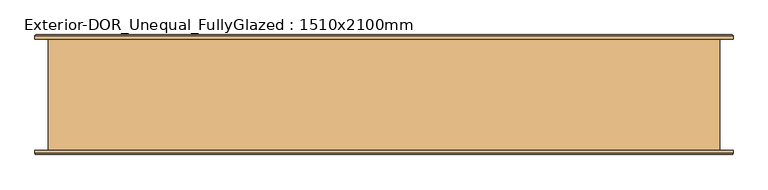
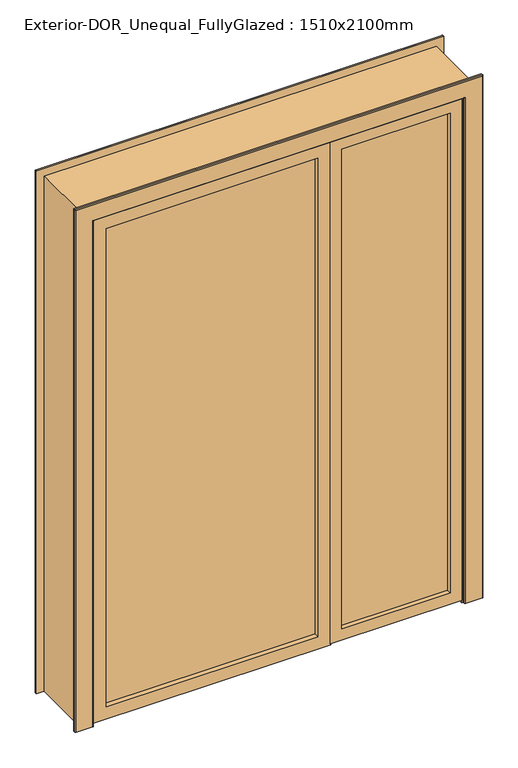
"""IFC4 building model written with IfcOpenShell, lengths in millimetres: door geometry, Exterior-DOR_Unequal_FullyGlazed : 1510x2100mm."""

from ifc_helpers import new_model, si_unit, frame, origin, place, context, project, spatial, polyline, circle_curve, ellipse_curve, outline, extrude, faceted_brep, source, transform, mapped, element, save
from ifc_brep_helpers import plane_surface, cylinder_surface, advanced_brep


def exterior_dor_unequal_fullyglazed_1510x2100mm_99816280(model_context):
    return source(origin(), model_context, "Body", "SolidModel", [
        extrude(outline(polyline([(247.5, -106.0), (247.5, -99.0), (665.0, -99.0), (665.0, -106.0), (247.5, -106.0)])), frame((0.0, 0.0, 55.0), z_axis=(0.0, 0.0, 1.0), x_axis=(1.0, 0.0, 0.0)), (0.0, 0.0, 1.0), 1955.0),
        extrude(outline(polyline([(10.0, 710.0), (2055.0, 710.0), (2055.0, 202.5), (10.0, 202.5), (10.0, 710.0)]), holes=[polyline([(2010.0, 247.5), (2010.0, 665.0), (55.0, 665.0), (55.0, 247.5), (2010.0, 247.5)])]), frame((0.0, -125.0, 0.0), z_axis=(0.0, 1.0, 0.0), x_axis=(0.0, 0.0, 1.0)), (0.0, 0.0, 1.0), 45.0),
        extrude(outline(polyline([(155.0, -106.0), (-660.0, -106.0), (-660.0, -99.0), (155.0, -99.0), (155.0, -106.0)])), frame((0.0, 0.0, 56.0), z_axis=(0.0, 0.0, 1.0), x_axis=(1.0, 0.0, 0.0)), (0.0, 0.0, 1.0), 1949.0),
        extrude(outline(polyline([(6.0, -710.0), (6.0, 205.0), (2055.0, 205.0), (2055.0, -710.0), (6.0, -710.0)]), holes=[polyline([(2005.0, 155.0), (56.0, 155.0), (56.0, -660.0), (2005.0, -660.0), (2005.0, 155.0)])]), frame((0.0, -125.0, 0.0), z_axis=(0.0, 1.0, 0.0), x_axis=(0.0, 0.0, 1.0)), (0.0, 0.0, 1.0), 45.0),
        advanced_brep(
        [(-715.0, -125.0, 0.0), (-715.0, -132.0, 0.0), (-718.0, -135.0, 0.0), (-782.0, -135.0, 0.0), (-785.0, -132.0, 0.0), (-785.0, -125.0, 0.0), (-715.0, -125.0, 2060.0), (-715.0, -132.0, 2060.0), (-718.0, -135.0, 2063.0), (718.0, -135.0, 2063.0), (718.0, -135.0, 0.0), (782.0, -135.0, 0.0), (782.0, -135.0, 2127.0), (-782.0, -135.0, 2127.0), (-785.0, -132.0, 2130.0), (-785.0, -125.0, 2130.0), (785.0, -125.0, 2130.0), (785.0, -125.0, 0.0), (715.0, -125.0, 0.0), (715.0, -125.0, 2060.0), (715.0, -132.0, 2060.0), (715.0, -132.0, 0.0), (785.0, -132.0, 0.0), (785.0, -132.0, 2130.0)],
        [
            (0, 1),
            (1, 2, circle_curve(frame((-718.0, -132.0, 0.0), z_axis=(0.0, 0.0, -1.0), x_axis=(-1.0, 0.0, 0.0)), 3.0)),
            (2, 3),
            (3, 4, circle_curve(frame((-782.0, -132.0, 0.0), z_axis=(0.0, 0.0, -1.0), x_axis=(-1.0, 0.0, 0.0)), 3.0)),
            (4, 5),
            (5, 0),
            (0, 6),
            (6, 7),
            (7, 1),
            (7, 8, ellipse_curve(frame((-718.0, -132.0, 2063.0), z_axis=(-0.7071067811865475, 0.0, -0.7071067811865475), x_axis=(0.7071067811865474, 0.0, -0.7071067811865476)), 4.2426407, 3.0)),
            (8, 2),
            (8, 9),
            (9, 10),
            (10, 11),
            (11, 12),
            (12, 13),
            (13, 3),
            (13, 14, ellipse_curve(frame((-782.0, -132.0, 2127.0), z_axis=(-0.7071067811865475, 0.0, -0.7071067811865475), x_axis=(0.7071067811865474, 0.0, -0.7071067811865476)), 4.2426407, 3.0)),
            (14, 4),
            (14, 15),
            (15, 5),
            (15, 16),
            (16, 17),
            (17, 18),
            (18, 19),
            (19, 6),
            (9, 20, ellipse_curve(frame((718.0, -132.0, 2063.0), z_axis=(0.7071067811865475, 0.0, -0.7071067811865475), x_axis=(0.7071067811865474, 0.0, 0.7071067811865476)), 4.2426407, 3.0)),
            (20, 21),
            (21, 10, circle_curve(frame((718.0, -132.0, 0.0), z_axis=(0.0, 0.0, 1.0), x_axis=(1.0, 0.0, 0.0)), 3.0)),
            (17, 22),
            (22, 11, circle_curve(frame((782.0, -132.0, 0.0), z_axis=(0.0, 0.0, -1.0), x_axis=(1.0, 0.0, 0.0)), 3.0)),
            (21, 18),
            (23, 12, ellipse_curve(frame((782.0, -132.0, 2127.0), z_axis=(0.7071067811865475, 0.0, -0.7071067811865475), x_axis=(0.7071067811865474, 0.0, 0.7071067811865476)), 4.2426407, 3.0)),
            (22, 23),
            (16, 23),
            (20, 19),
            (20, 7),
            (23, 14),
        ],
        [
            plane_surface(frame((-755.0, 125.0, 0.0), z_axis=(0.0, 0.0, -1.0), x_axis=(0.0, -1.0, 0.0))),
            plane_surface(frame((-715.0, -125.0, 0.0), z_axis=(1.0, 0.0, 0.0), x_axis=(0.0, 0.0, 1.0))),
            cylinder_surface(frame((-718.0, -132.0, 0.0), z_axis=(0.0, 0.0, -1.0), x_axis=(-1.0, 0.0, 0.0)), 3.0),
            plane_surface(frame((-718.0, -135.0, 0.0), z_axis=(0.0, -1.0, 0.0), x_axis=(0.0, 0.0, 1.0))),
            cylinder_surface(frame((-782.0, -132.0, 0.0), z_axis=(0.0, 0.0, -1.0), x_axis=(-1.0, 0.0, 0.0)), 3.0),
            plane_surface(frame((-785.0, -132.0, 0.0), z_axis=(-1.0, 0.0, 0.0), x_axis=(0.0, 0.0, 1.0))),
            plane_surface(frame((-785.0, -125.0, 0.0), z_axis=(0.0, 1.0, 0.0), x_axis=(0.0, 0.0, 1.0))),
            cylinder_surface(frame((718.0, -132.0, 2100.0), z_axis=(0.0, 0.0, 1.0), x_axis=(1.0, 0.0, 0.0)), 3.0),
            plane_surface(frame((755.0, 125.0, 0.0), z_axis=(0.0, 0.0, -1.0), x_axis=(0.0, -1.0, 0.0))),
            cylinder_surface(frame((782.0, -132.0, 2100.0), z_axis=(0.0, 0.0, 1.0), x_axis=(1.0, 0.0, 0.0)), 3.0),
            plane_surface(frame((785.0, -132.0, 2130.0), z_axis=(1.0, 0.0, 0.0), x_axis=(0.0, 0.0, -1.0))),
            plane_surface(frame((715.0, -125.0, 2060.0), z_axis=(-1.0, 0.0, 0.0), x_axis=(0.0, 0.0, -1.0))),
            plane_surface(frame((-715.0, -125.0, 2060.0), z_axis=(0.0, 0.0, -1.0), x_axis=(1.0, 0.0, 0.0))),
            cylinder_surface(frame((-755.0, -132.0, 2063.0), z_axis=(-1.0, 0.0, 0.0), x_axis=(0.0, 0.0, 1.0)), 3.0),
            cylinder_surface(frame((-755.0, -132.0, 2127.0), z_axis=(-1.0, 0.0, 0.0), x_axis=(0.0, 0.0, 1.0)), 3.0),
            plane_surface(frame((-785.0, -132.0, 2130.0), z_axis=(0.0, 0.0, 1.0), x_axis=(1.0, 0.0, 0.0))),
        ],
        [
            (0, [[1, 2, 3, 4, 5, 6]]),
            (1, [[-1, 7, 8, 9]]),
            (2, [[-2, -9, 10, 11]]),
            (3, [[-3, -11, 12, 13, 14, 15, 16, 17]]),
            (4, [[-4, -17, 18, 19]]),
            (5, [[-5, -19, 20, 21]]),
            (6, [[-6, -21, 22, 23, 24, 25, 26, -7]]),
            (7, [[27, 28, 29, -13]]),
            (8, [[-24, 30, 31, -14, -29, 32]]),
            (9, [[33, -15, -31, 34]]),
            (10, [[35, -34, -30, -23]]),
            (11, [[36, -25, -32, -28]]),
            (12, [[-8, -26, -36, 37]]),
            (13, [[-10, -37, -27, -12]]),
            (14, [[-18, -16, -33, 38]]),
            (15, [[-20, -38, -35, -22]]),
        ],
    ),
        advanced_brep(
        [(-785.0, 125.0, 0.0), (-785.0, 132.0, 0.0), (-782.0, 135.0, 0.0), (-718.0, 135.0, 0.0), (-715.0, 132.0, 0.0), (-715.0, 125.0, 0.0), (-785.0, 125.0, 2130.0), (-785.0, 132.0, 2130.0), (-782.0, 135.0, 2127.0), (782.0, 135.0, 2127.0), (782.0, 135.0, 0.0), (718.0, 135.0, 0.0), (718.0, 135.0, 2063.0), (-718.0, 135.0, 2063.0), (-715.0, 132.0, 2060.0), (-715.0, 125.0, 2060.0), (715.0, 125.0, 2060.0), (715.0, 125.0, 0.0), (785.0, 125.0, 0.0), (785.0, 125.0, 2130.0), (785.0, 132.0, 2130.0), (785.0, 132.0, 0.0), (715.0, 132.0, 0.0), (715.0, 132.0, 2060.0)],
        [
            (0, 1),
            (1, 2, circle_curve(frame((-782.0, 132.0, 0.0), z_axis=(0.0, 0.0, -1.0), x_axis=(-1.0, 0.0, 0.0)), 3.0)),
            (2, 3),
            (3, 4, circle_curve(frame((-718.0, 132.0, 0.0), z_axis=(0.0, 0.0, -1.0), x_axis=(-1.0, 0.0, 0.0)), 3.0)),
            (4, 5),
            (5, 0),
            (0, 6),
            (6, 7),
            (7, 1),
            (7, 8, ellipse_curve(frame((-782.0, 132.0, 2127.0), z_axis=(-0.7071067811865475, 0.0, -0.7071067811865475), x_axis=(0.7071067811865474, 0.0, -0.7071067811865476)), 4.2426407, 3.0)),
            (8, 2),
            (8, 9),
            (9, 10),
            (10, 11),
            (11, 12),
            (12, 13),
            (13, 3),
            (13, 14, ellipse_curve(frame((-718.0, 132.0, 2063.0), z_axis=(-0.7071067811865475, 0.0, -0.7071067811865475), x_axis=(0.7071067811865474, 0.0, -0.7071067811865476)), 4.2426407, 3.0)),
            (14, 4),
            (14, 15),
            (15, 5),
            (15, 16),
            (16, 17),
            (17, 18),
            (18, 19),
            (19, 6),
            (9, 20, ellipse_curve(frame((782.0, 132.0, 2127.0), z_axis=(0.7071067811865475, 0.0, -0.7071067811865475), x_axis=(0.7071067811865474, 0.0, 0.7071067811865476)), 4.2426407, 3.0)),
            (20, 21),
            (21, 10, circle_curve(frame((782.0, 132.0, 0.0), z_axis=(0.0, 0.0, 1.0), x_axis=(1.0, 0.0, 0.0)), 3.0)),
            (17, 22),
            (22, 11, circle_curve(frame((718.0, 132.0, 0.0), z_axis=(0.0, 0.0, -1.0), x_axis=(1.0, 0.0, 0.0)), 3.0)),
            (21, 18),
            (23, 12, ellipse_curve(frame((718.0, 132.0, 2063.0), z_axis=(0.7071067811865475, 0.0, -0.7071067811865475), x_axis=(0.7071067811865474, 0.0, 0.7071067811865476)), 4.2426407, 3.0)),
            (22, 23),
            (16, 23),
            (20, 19),
            (20, 7),
            (23, 14),
        ],
        [
            plane_surface(frame((-755.0, 125.0, 0.0), z_axis=(0.0, 0.0, -1.0), x_axis=(0.0, -1.0, 0.0))),
            plane_surface(frame((-785.0, 125.0, 0.0), z_axis=(-1.0, 0.0, 0.0), x_axis=(0.0, 0.0, 1.0))),
            cylinder_surface(frame((-782.0, 132.0, 0.0), z_axis=(0.0, 0.0, -1.0), x_axis=(-1.0, 0.0, 0.0)), 3.0),
            plane_surface(frame((-782.0, 135.0, 0.0), z_axis=(0.0, 1.0, 0.0), x_axis=(0.0, 0.0, 1.0))),
            cylinder_surface(frame((-718.0, 132.0, 0.0), z_axis=(0.0, 0.0, -1.0), x_axis=(-1.0, 0.0, 0.0)), 3.0),
            plane_surface(frame((-715.0, 132.0, 0.0), z_axis=(1.0, 0.0, 0.0), x_axis=(0.0, 0.0, 1.0))),
            plane_surface(frame((-715.0, 125.0, 0.0), z_axis=(0.0, -1.0, 0.0), x_axis=(0.0, 0.0, 1.0))),
            cylinder_surface(frame((782.0, 132.0, 2100.0), z_axis=(0.0, 0.0, 1.0), x_axis=(1.0, 0.0, 0.0)), 3.0),
            plane_surface(frame((755.0, 125.0, 0.0), z_axis=(0.0, 0.0, -1.0), x_axis=(0.0, -1.0, 0.0))),
            cylinder_surface(frame((718.0, 132.0, 2100.0), z_axis=(0.0, 0.0, 1.0), x_axis=(1.0, 0.0, 0.0)), 3.0),
            plane_surface(frame((715.0, 132.0, 2060.0), z_axis=(-1.0, 0.0, 0.0), x_axis=(0.0, 0.0, -1.0))),
            plane_surface(frame((785.0, 125.0, 2130.0), z_axis=(1.0, 0.0, 0.0), x_axis=(0.0, 0.0, -1.0))),
            plane_surface(frame((-785.0, 125.0, 2130.0), z_axis=(0.0, 0.0, 1.0), x_axis=(1.0, 0.0, 0.0))),
            cylinder_surface(frame((-755.0, 132.0, 2127.0), z_axis=(-1.0, 0.0, 0.0), x_axis=(0.0, 0.0, 1.0)), 3.0),
            cylinder_surface(frame((-755.0, 132.0, 2063.0), z_axis=(-1.0, 0.0, 0.0), x_axis=(0.0, 0.0, 1.0)), 3.0),
            plane_surface(frame((-715.0, 132.0, 2060.0), z_axis=(0.0, 0.0, -1.0), x_axis=(1.0, 0.0, 0.0))),
        ],
        [
            (0, [[1, 2, 3, 4, 5, 6]]),
            (1, [[-1, 7, 8, 9]]),
            (2, [[-2, -9, 10, 11]]),
            (3, [[-3, -11, 12, 13, 14, 15, 16, 17]]),
            (4, [[-4, -17, 18, 19]]),
            (5, [[-5, -19, 20, 21]]),
            (6, [[-6, -21, 22, 23, 24, 25, 26, -7]]),
            (7, [[27, 28, 29, -13]]),
            (8, [[-24, 30, 31, -14, -29, 32]]),
            (9, [[33, -15, -31, 34]]),
            (10, [[35, -34, -30, -23]]),
            (11, [[36, -25, -32, -28]]),
            (12, [[-8, -26, -36, 37]]),
            (13, [[-10, -37, -27, -12]]),
            (14, [[-18, -16, -33, 38]]),
            (15, [[-20, -38, -35, -22]]),
        ],
    ),
        faceted_brep([(-755.0, 125.0, 0.0), (-710.0, 125.0, 0.0), (-710.0, -40.0, 0.0), (-690.0, -40.0, 0.0), (-690.0, -80.0, 0.0), (-710.0, -80.0, 0.0), (-710.0, -125.0, 0.0), (-755.0, -125.0, 0.0), (-755.0, 125.0, 2100.0), (755.0, 125.0, 2100.0), (755.0, 125.0, 0.0), (710.0, 125.0, 0.0), (710.0, 125.0, 2055.0), (-710.0, 125.0, 2055.0), (-710.0, -40.0, 2055.0), (710.0, -40.0, 2055.0), (710.0, -40.0, 0.0), (690.0, -40.0, 0.0), (690.0, -40.0, 2035.0), (-690.0, -40.0, 2035.0), (-690.0, -80.0, 2035.0), (690.0, -80.0, 2035.0), (690.0, -80.0, 0.0), (710.0, -80.0, 0.0), (710.0, -80.0, 2055.0), (-710.0, -80.0, 2055.0), (-710.0, -125.0, 2055.0), (710.0, -125.0, 2055.0), (710.0, -125.0, 0.0), (755.0, -125.0, 0.0), (755.0, -125.0, 2100.0), (-755.0, -125.0, 2100.0)], [[[0, 1, 2, 3, 4, 5, 6, 7]], [[1, 0, 8, 9, 10, 11, 12, 13]], [[2, 1, 13, 14]], [[3, 2, 14, 15, 16, 17, 18, 19]], [[4, 3, 19, 20]], [[5, 4, 20, 21, 22, 23, 24, 25]], [[6, 5, 25, 26]], [[7, 6, 26, 27, 28, 29, 30, 31]], [[0, 7, 31, 8]], [[9, 30, 29, 10]], [[10, 29, 28, 23, 22, 17, 16, 11]], [[15, 12, 11, 16]], [[21, 18, 17, 22]], [[27, 24, 23, 28]], [[20, 19, 18, 21]], [[26, 25, 24, 27]], [[8, 31, 30, 9]], [[14, 13, 12, 15]]]),
    ])


if __name__ == "__main__":
    model = new_model("IFC4")
    model_context = context("Model", 3, world=origin())
    ifc_project = project(units=[si_unit("LENGTHUNIT", "METRE", prefix="MILLI")], contexts=[model_context])
    site = spatial("IfcSite", under=ifc_project)
    building = spatial("IfcBuilding", under=site)
    placement = place(None, origin())
    exterior_dor_unequal_fullyglazed_1510x2100mm_shape = exterior_dor_unequal_fullyglazed_1510x2100mm_99816280(model_context)
    element("IfcDoor", 1, ObjectType="Exterior-DOR_Unequal_FullyGlazed : 1510x2100mm", at=placement, inside=building, context=model_context, shape_type="MappedRepresentation", body=[
        mapped(exterior_dor_unequal_fullyglazed_1510x2100mm_shape, transform((0.0, 0.0, 0.0), x_axis=(1.0, 0.0, 0.0), y_axis=(0.0, 1.0, 0.0), z_axis=(0.0, 0.0, 1.0))),
    ])
    save(model, "model.ifc")

# Revit data of these elements
# Type "Exterior-DOR_Unequal_FullyGlazed : 1510x2100mm"
#   Type IfcGUID = "2NKTNbJKP36hSTtB23uCk3"
#   Assembly Code = "B2030100"
#   Type Mark = "190"
#   Classification.Uniclass.EF.Number = "EF_25_30"
#   Classification.Uniclass.EF.Description = "Doors and windows"
#   WindLoadRating = "n/a"
#   WaterTightnessRating = "n/a"
#   WarrantyStartDate [instance default] = "1900-12-31T23:59:59"
#   WarrantyGuarantorParts = "n/a"
#   WarrantyGuarantorLabor = "n/a"
#   WarrantyDurationUnit = "year"
#   WarrantyDurationParts = "n/a"
#   WarrantyDurationLabor = "n/a"
#   WarrantyDescription = "n/a"
#   Version = "2"
#   Uniclass2015Version = "Systems v1.9"
#   Uniclass2015Title = "Doorset systems"
#   Uniclass2015Code = "Ss_25_30_20_25"
#   URL = "www.nationalbimlibrary.com"
#   TagNumber [instance default] = "n/a"
#   SustainabilityPerformance = "n/a"
#   Status = "UNSET"
#   Size = "1510 x 2100 mm"
#   Shape = "n/a"
#   SerialNumber [instance default] = "n/a"
#   SecurityRating = "n/a"
#   Revision = "n/a"
#   ReplacementCost = "n/a"
#   Reference = "n/a"
#   ProductInformation = "n/a"
#   Operation = "DOUBLE_DOOR_SINGLE_SWING"
#   OmniClassVersion = "Table 22 2012-05-16"
#   OmniClassTitle = "Doors and Frames"
#   OmniClassCode = "22-08 10 00"
#   Name = "DoorsetSystem_Interior-Unequal_FullGlazed"
#   NBSReference = "25-50-20/120"
#   NBSDescription = "Doorset system"
#   NBSCertification = "www.nationalbimlibrary.com/cert/fxtqd0eu"
#   ModelReference = "Interior Unequal Door Fully Glazed Leaf"
#   ModelNumber = "n/a"
#   Model = "Interior Unequal Door Fully Glazed Leaf"
#   MechanicalLoadRating = "n/a"
#   Material = "n/a"
#   ManufacturerURL = "n/a"
#   ManufacturerName = "n/a"
#   Manufacturer = "info@theNBS.com"
#   InstallationDate [instance default] = "1900-12-31T23:59:59"
#   IfcExportType = "DOOR"
#   IfcExportAs = "IfcDoorType"
#   HygrothermalRating = "n/a"
#   Grade = "n/a"
#   GlassColor = "n/a"
#   FireRating = "n/a"
#   Fire Rating = "n/a"
#   Finish = "n/a"
#   FillGas = "n/a"
#   Features = "n/a"
#   ExpectedLife = "n/a"
#   DurationUnit = "n/a"
#   DurabilityRating = "n/a"
#   DoorNumber [instance default] = "n/a"
#   Description = "Generic unequal interior door with fully glazed leaf"
#   Construction Type = "ALUMINIUM"
#   Constituents = "n/a"
#   ComponentNumber [instance default] = "n/a"
#   Color = "n/a"
#   CodePerformance = "n/a"
#   Category = "Ss_25_30_20_25:Doorset systems"
#   BarCode [instance default] = "n/a"
#   BIMObjectName = "NBS_DoorsetSystem_Interior-Unequal_FullyGlazed"
#   Author = "NBS"
#   AssetType = "Fixed"
#   AssetIdentifier [instance default] = "n/a"
#   Analytic Construction = "<None>"
#   AcousticRating = "n/a"
#   AccessibilityPerformance = "n/a"
#   Width = 1.51 m
#   WallThickness [instance default] = 0.15 m
#   VisibleLightTransmittance = 0
#   VisibileLightReflectance = 0
#   Thickness = 0.15 m
#   ThermalTransmittanceWinter = 0
#   ThermalTransmittanceSummer = 0
#   ThermalTransmittance = 0
#   StructuralToleranceJamb = 0 m
#   StructuralToleranceHead = 0 m
#   StructuralOpeningWidth = 1.51 m
#   StructuralOpeningHeight = 2.1 m
#   StopProjection = 0.02 m
#   StopDepth = 0.04 m
#   SolarTransmittance = 0
#   SolarReflectance = 0
#   SolarHeatGainTransmittance = 0
#   SolarAbsorption = 0
#   ShadingCoefficient = 0
#   SecondaryPanelWidth = 0.5075 m
#   Rough Width [instance default] = 1.51 m
#   Rough Height [instance default] = 2.1 m
#   RebateDepth = 0.045 m
#   PanelUndercut = 0.006 m
#   PanelHeight = 2.055 m
#   PanelDepth = 0.045 m
#   OpeningTolerance = 0 m
#   NominalWidth = 1.51 m
#   NominalLength = 0 m
#   NominalHeight = 2.1 m
#   MeetingStileTolerance = 0.0025 m
#   MainPanelWidth = 0.91 m
#   Infiltration = 0
#   Height = 2.1 m
#   GlazingPanelWidth = 0.2 m
#   GlazingPanelThickness = 0.007 m
#   GlazingPanelDiameter = 0.4 m
#   GlazingPanelCentre = 1.6 m
#   GlazingOffsetFromEdgeOfPanel = 0.2 m
#   GlazingOffsetFromBottomOfPanel = 1.106 m
#   GlazingAreaFraction = 0
#   GlassThickness3 = 0.002 m
#   GlassThickness2 = 0.002 m
#   GlassThickness1 = 0.002 m
#   FrameThickness = 0.045 m
#   FrameSetback [instance default] = 0 m
#   FrameDepth [instance default] = 0.15 m
#   FinishThicknessInternal [instance default] = 0 m
#   FinishThicknessExternal [instance default] = 0 m
#   ClearOpeningWidth = 1.38 m
#   ClearOpeningHeight = 2.035 m
#   CalculatedInteriorVoidDepth [instance default] = 0.3 m
#   ArchitraveWidth = 0.07 m
#   ArchitraveThickness = 0.01 m
#   ArchitraveSetbackFromFrameFace = 0.005 m
#   SmokeStop = no
#   SingleRebate = no
#   SelfClosing = no
#   PlantedStop = yes
#   IsWired = no
#   IsTempered = no
#   IsLaminated = no
#   IsExternal = yes
#   IsCoated = no
#   HasDrive = no
#   HandicapAccessible = no
#   GlassLayers = 3
#   Function = 1
#   Wall Closure = 4
#   FireExit = no
#   ArchitraveFrontRequired [instance default] = yes
#   ArchitraveBackRequired [instance default] = yes
#   PanelMaterial = NBS_Concept
#   GlazingPanelMaterial = NBS_Glass_Single
#   GlazingBeadMaterial = NBS_Concept
#   FrameSectionMaterial = NBS_Concept
#   Cost = 0
# Element 1 (IfcDoor, "Exterior-DOR_Unequal_FullyGlazed : 1510x2100mm")
#   WallThickness = 0.25 m
#   FrameDepth = 0.25 m
#   Materials on its faces: "NBS_Concept", "NBS_Glass_Single"
# Materials
#   "NBS_Concept": class "Generic", colour RGB 255 255 255, transparency 0, Description = "To be specified", Cost = 0
#   "NBS_Glass_Single": class "Glass", colour RGB 94 140 251, transparency 0.6, Cost = 0
